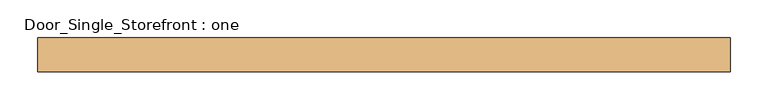
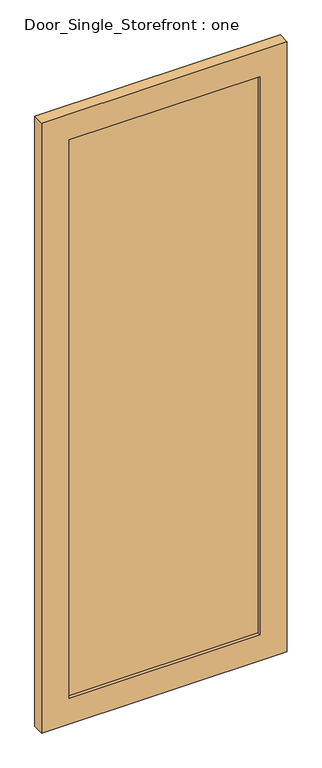
"""IFC4 building model written with IfcOpenShell, lengths in millimetres: door geometry, Door_Single_Storefront : one."""

from ifc_helpers import new_model, si_unit, frame, origin, place, context, project, spatial, polyline, outline, extrude, source, transform, mapped, element, save


def door_single_storefront_one_a6b5570d(model_context):
    return source(origin(), model_context, "Body", "SweptSolid", [
        extrude(outline(polyline([(355.6, 6.35), (355.6, -12.7), (-355.6, -12.7), (-355.6, 6.35), (355.6, 6.35)])), frame((0.0, 0.0, 101.6), z_axis=(0.0, 0.0, 1.0), x_axis=(1.0, 0.0, 0.0)), (0.0, 0.0, 1.0), 2197.1),
        extrude(outline(polyline([(2400.3, -457.2), (0.0, -457.2), (0.0, 457.2), (2400.3, 457.2), (2400.3, -457.2)]), holes=[polyline([(101.6, 355.6), (101.6, -355.6), (2298.7, -355.6), (2298.7, 355.6), (101.6, 355.6)])]), frame((0.0, -25.4, 0.0), z_axis=(0.0, 1.0, 0.0), x_axis=(0.0, 0.0, 1.0)), (0.0, 0.0, 1.0), 44.45),
    ])


if __name__ == "__main__":
    model = new_model("IFC4")
    model_context = context("Model", 3, world=origin())
    ifc_project = project(units=[si_unit("LENGTHUNIT", "METRE", prefix="MILLI")], contexts=[model_context])
    site = spatial("IfcSite", under=ifc_project)
    building = spatial("IfcBuilding", under=site)
    placement = place(None, origin())
    door_single_storefront_one_shape = door_single_storefront_one_a6b5570d(model_context)
    element("IfcDoor", 1, ObjectType="Door_Single_Storefront : one", at=placement, inside=building, context=model_context, shape_type="MappedRepresentation", body=[
        mapped(door_single_storefront_one_shape, transform((0.0, 0.0, 0.0), x_axis=(1.0, 0.0, 0.0), y_axis=(0.0, 1.0, 0.0), z_axis=(0.0, 0.0, 1.0))),
    ])
    save(model, "model.ifc")

# Revit data of these elements
# Type "Door_Single_Storefront : one"
#   Type Mark = "27"
#   Analytic Construction = "<None>"
#   Stile_Width = 0' - 4"
#   Door_Thickness = 0' - 1 3/4"
#   Door_Offset = 0' - 1"
#   Glass_Material = Glass
#   Frame_Material = Aluminum
#   Function = (empty or 0)
# Element 1 (IfcDoor, "Door_Single_Storefront : one")
#   Materials on its faces: "Aluminum", "Glass"
# Materials
#   "Glass": class "Glass", colour RGB 142 168 196, transparency 0.75, Description = "Soda Lime Glass", Cost = 0
#   "Aluminum": class "Metal", colour RGB 226 226 226, transparency 0, Description = "Aluminum 6061", Cost = 0
